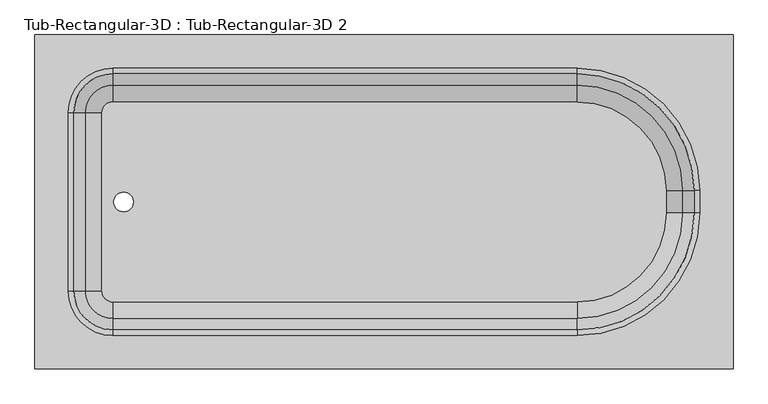
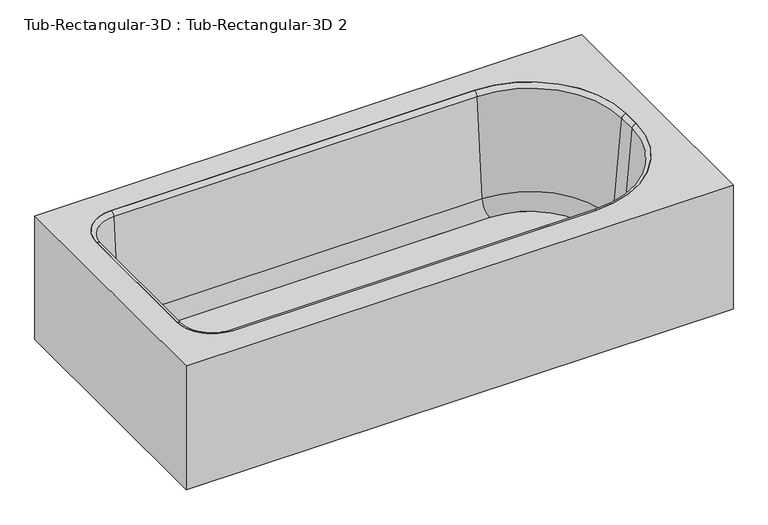
"""IFC4 building model written with IfcOpenShell, lengths in millimetres: flow terminal geometry, Tub-Rectangular-3D : Tub-Rectangular-3D 2."""

from ifc_helpers import new_model, si_unit, point, frame, frame_2d, origin, place, context, project, spatial, polyline, circle_curve, ellipse_curve, trimmed, segment, composite_curve, outline, extrude, source, transform, mapped, element, save
from ifc_brep_helpers import plane_surface, cylinder_surface, revolved_surface, advanced_brep


def tub_rectangular_3d_tub_rectangular_3d_2_4c7bd2b7(model_context):
    return source(origin(), model_context, "Body", "SolidModel", [
        advanced_brep(
        [(480.0720313, 866.775, 381.0), (-1110.6029687, 866.775, 381.0), (-1110.6029687, 104.775, 381.0), (480.0720313, 104.775, 381.0), (-932.8029687, 790.575, 381.0), (124.4720313, 790.575, 381.0), (403.8720313, 511.175, 381.0), (403.8720313, 460.375, 381.0), (124.4720313, 180.975, 381.0), (-932.8029687, 180.975, 381.0), (-1034.4029687, 282.575, 381.0), (-1034.4029687, 688.975, 381.0), (461.0220313, 847.725, 361.95), (461.0220313, 123.825, 361.95), (-1091.5529687, 123.825, 361.95), (-1091.5529687, 847.725, 361.95), (-932.8029687, 790.575, 361.95), (-1034.4029687, 688.975, 361.95), (-1034.4029687, 282.575, 361.95), (-932.8029687, 180.975, 361.95), (124.4720313, 180.975, 361.95), (403.8720313, 460.375, 361.95), (403.8720313, 511.175, 361.95), (124.4720313, 790.575, 361.95), (480.0720313, 866.775, 0.0), (-1110.6029687, 866.775, 0.0), (-1110.6029687, 104.775, 0.0), (480.0720313, 104.775, 0.0), (461.0220313, 847.725, 0.0), (-1091.5529687, 847.725, 0.0), (-1091.5529687, 123.825, 0.0), (461.0220313, 123.825, 0.0)],
        [
            (0, 1),
            (1, 2),
            (2, 3),
            (3, 0),
            (4, 5),
            (5, 6, circle_curve(frame((124.4720313, 511.175, 381.0), z_axis=(0.0, 0.0, -1.0), x_axis=(0.0, 1.0, 0.0)), 279.4)),
            (6, 7),
            (7, 8, circle_curve(frame((124.4720313, 460.375, 381.0), z_axis=(0.0, 0.0, -1.0), x_axis=(0.0, 1.0, 0.0)), 279.4)),
            (8, 9),
            (9, 10, circle_curve(frame((-932.8029687, 282.575, 381.0), z_axis=(0.0, 0.0, -1.0), x_axis=(0.0, 1.0, 0.0)), 101.6)),
            (10, 11),
            (11, 4, circle_curve(frame((-932.8029687, 688.975, 381.0), z_axis=(0.0, 0.0, -1.0), x_axis=(0.0, 1.0, 0.0)), 101.6)),
            (12, 13),
            (13, 14),
            (14, 15),
            (15, 12),
            (16, 17, circle_curve(frame((-932.8029687, 688.975, 361.95), z_axis=(0.0, 0.0, 1.0), x_axis=(0.0, 1.0, 0.0)), 101.6)),
            (17, 18),
            (18, 19, circle_curve(frame((-932.8029687, 282.575, 361.95), z_axis=(0.0, 0.0, 1.0), x_axis=(0.0, 1.0, 0.0)), 101.6)),
            (19, 20),
            (20, 21, circle_curve(frame((124.4720313, 460.375, 361.95), z_axis=(0.0, 0.0, 1.0), x_axis=(0.0, 1.0, 0.0)), 279.4)),
            (21, 22),
            (22, 23, circle_curve(frame((124.4720313, 511.175, 361.95), z_axis=(0.0, 0.0, 1.0), x_axis=(0.0, 1.0, 0.0)), 279.4)),
            (23, 16),
            (0, 24),
            (24, 25),
            (25, 1),
            (25, 26),
            (26, 2),
            (26, 27),
            (27, 3),
            (27, 24),
            (4, 16),
            (23, 5),
            (22, 6),
            (21, 7),
            (20, 8),
            (19, 9),
            (18, 10),
            (17, 11),
            (28, 29),
            (29, 30),
            (30, 31),
            (31, 28),
            (31, 13),
            (12, 28),
            (30, 14),
            (29, 15),
        ],
        [
            plane_surface(frame((-1110.6029687, 866.775, 381.0), z_axis=(0.0, 0.0, 1.0), x_axis=(-1.0, 0.0, 0.0))),
            plane_surface(frame((-1110.6029687, 866.775, 361.95), z_axis=(0.0, 0.0, -1.0), x_axis=(1.0, 0.0, 0.0))),
            plane_surface(frame((480.0720313, 866.775, 381.0), z_axis=(0.0, 1.0, 0.0), x_axis=(0.0, 0.0, -1.0))),
            plane_surface(frame((-1110.6029687, 866.775, 381.0), z_axis=(-1.0, 0.0, 0.0), x_axis=(0.0, 0.0, -1.0))),
            plane_surface(frame((-1110.6029687, 104.775, 381.0), z_axis=(0.0, -1.0, 0.0), x_axis=(0.0, 0.0, -1.0))),
            plane_surface(frame((480.0720313, 104.775, 381.0), z_axis=(1.0, 0.0, 0.0), x_axis=(0.0, 0.0, -1.0))),
            plane_surface(frame((-932.8029687, 790.575, 381.0), z_axis=(0.0, -1.0, 0.0), x_axis=(0.0, 0.0, -1.0))),
            revolved_surface(polyline([(124.4720313, 790.575, 361.95), (124.4720313, 790.575, 381.0)]), (124.4720313, 511.175, 381.0), (0.0, 0.0, -1.0)),
            plane_surface(frame((403.8720313, 511.175, 381.0), z_axis=(-1.0, 0.0, 0.0), x_axis=(0.0, 0.0, -1.0))),
            revolved_surface(polyline([(124.4720313, 739.775, 361.95), (124.4720313, 739.775, 381.0)]), (124.4720313, 460.375, 381.0), (0.0, 0.0, -1.0)),
            plane_surface(frame((124.4720313, 180.975, 381.0), z_axis=(0.0, 1.0, 0.0), x_axis=(0.0, 0.0, -1.0))),
            revolved_surface(polyline([(-932.8029687, 384.17499999999995, 361.95), (-932.8029687, 384.17499999999995, 381.0)]), (-932.8029687, 282.575, 381.0), (0.0, 0.0, -1.0)),
            plane_surface(frame((-1034.4029687, 282.575, 381.0), z_axis=(1.0, 0.0, 0.0), x_axis=(0.0, 0.0, -1.0))),
            revolved_surface(polyline([(-932.8029687, 790.575, 361.95), (-932.8029687, 790.575, 381.0)]), (-932.8029687, 688.975, 381.0), (0.0, 0.0, -1.0)),
            plane_surface(frame((-1110.6029687, 866.775, 0.0), z_axis=(0.0, 0.0, -1.0), x_axis=(1.0, 0.0, 0.0))),
            plane_surface(frame((461.0220313, 847.725, 361.95), z_axis=(-1.0, 0.0, 0.0), x_axis=(0.0, 0.0, -1.0))),
            plane_surface(frame((461.0220313, 123.825, 361.95), z_axis=(0.0, 1.0, 0.0), x_axis=(0.0, 0.0, -1.0))),
            plane_surface(frame((-1091.5529687, 123.825, 361.95), z_axis=(1.0, 0.0, 0.0), x_axis=(0.0, 0.0, -1.0))),
            plane_surface(frame((-1091.5529687, 847.725, 361.95), z_axis=(0.0, -1.0, 0.0), x_axis=(0.0, 0.0, -1.0))),
        ],
        [
            (0, [[1, 2, 3, 4], [5, 6, 7, 8, 9, 10, 11, 12]]),
            (1, [[13, 14, 15, 16], [17, 18, 19, 20, 21, 22, 23, 24]]),
            (2, [[-1, 25, 26, 27]]),
            (3, [[-2, -27, 28, 29]]),
            (4, [[-3, -29, 30, 31]]),
            (5, [[-25, -4, -31, 32]]),
            (6, [[-5, 33, -24, 34]]),
            (7, [[-6, -34, -23, 35]]),
            (8, [[-7, -35, -22, 36]]),
            (9, [[-8, -36, -21, 37]]),
            (10, [[-9, -37, -20, 38]]),
            (11, [[-10, -38, -19, 39]]),
            (12, [[-11, -39, -18, 40]]),
            (13, [[-12, -40, -17, -33]]),
            (14, [[-32, -30, -28, -26], [41, 42, 43, 44]]),
            (15, [[-44, 45, -13, 46]]),
            (16, [[-43, 47, -14, -45]]),
            (17, [[-42, 48, -15, -47]]),
            (18, [[-41, -46, -16, -48]]),
        ],
    ),
        extrude(outline(composite_curve([segment(trimmed(circle_curve(frame_2d((124.4720313, 511.175)), 202.7964741), [point((124.4720313, 713.9714741))], [point((327.2685054, 511.175))], False, "CARTESIAN"), True, "CONTINUOUS"), segment(polyline([(327.2685054, 511.175), (327.2685054, 460.375)]), True, "CONTINUOUS"), segment(trimmed(circle_curve(frame_2d((124.4720313, 460.375)), 202.7964741), [point((327.2685054, 460.375))], [point((124.4720313, 257.5785259))], False, "CARTESIAN"), True, "CONTINUOUS"), segment(polyline([(124.4720313, 257.5785259), (-932.8029687, 257.5785259)]), True, "CONTINUOUS"), segment(trimmed(circle_curve(frame_2d((-932.8029687, 282.575)), 24.9964741), [point((-932.8029687, 257.5785259))], [point((-957.7994428, 282.575))], False, "CARTESIAN"), True, "CONTINUOUS"), segment(polyline([(-957.7994428, 282.575), (-957.7994428, 688.975)]), True, "CONTINUOUS"), segment(trimmed(circle_curve(frame_2d((-932.8029687, 688.975)), 24.9964741), [point((-957.7994428, 688.975))], [point((-932.8029687, 713.9714741))], False, "CARTESIAN"), True, "CONTINUOUS"), segment(polyline([(-932.8029687, 713.9714741), (124.4720313, 713.9714741)]), True, "CONTINUOUS")], self_intersect=False), holes=[composite_curve([segment(trimmed(circle_curve(frame_2d((-908.510206, 485.775)), 22.225), [point((-908.510206, 508.0))], [point((-908.510206, 463.55))], True, "CARTESIAN"), True, "CONTINUOUS"), segment(trimmed(circle_curve(frame_2d((-908.510206, 485.775)), 22.225), [point((-908.510206, 463.55))], [point((-908.510206, 508.0))], True, "CARTESIAN"), True, "CONTINUOUS")], self_intersect=False)]), frame((0.0, 0.0, 16.863573), z_axis=(0.0, 0.0, 1.0), x_axis=(1.0, 0.0, 0.0)), (0.0, 0.0, 1.0), 19.05),
        advanced_brep(
        [(-995.7544608, 688.975, 70.6929392), (-932.8029687, 751.9264921, 70.6929392), (-932.8029687, 778.0970035, 369.8232535), (-1021.9249722, 688.975, 369.8232535), (-957.7994428, 688.975, 35.913573), (-932.8029687, 713.9714741, 35.913573), (-957.7994428, 688.975, 16.863573), (-932.8029687, 713.9714741, 16.863573), (-1034.4029687, 688.975, 16.863573), (-932.8029687, 790.575, 16.863573), (-1034.4029687, 688.975, 381.0), (-932.8029687, 790.575, 381.0), (-1021.9249722, 282.575, 369.8232535), (-995.7544608, 282.575, 70.6929392), (-957.7994428, 282.575, 35.913573), (-957.7994428, 282.575, 16.863573), (-1034.4029687, 282.575, 16.863573), (-1034.4029687, 282.575, 381.0), (-932.8029687, 219.6235079, 70.6929392), (-932.8029687, 193.4529965, 369.8232535), (-932.8029687, 257.5785259, 35.913573), (-932.8029687, 257.5785259, 16.863573), (-932.8029687, 180.975, 16.863573), (-932.8029687, 180.975, 381.0), (124.4720313, 193.4529965, 369.8232535), (124.4720313, 219.6235079, 70.6929392), (124.4720313, 257.5785259, 35.913573), (124.4720313, 257.5785259, 16.863573), (124.4720313, 180.975, 16.863573), (124.4720313, 180.975, 381.0), (365.2235234, 460.375, 70.6929392), (391.3940348, 460.375, 369.8232535), (327.2685054, 460.375, 35.913573), (327.2685054, 460.375, 16.863573), (403.8720313, 460.375, 16.863573), (403.8720313, 460.375, 381.0), (391.3940348, 511.175, 369.8232535), (365.2235234, 511.175, 70.6929392), (327.2685054, 511.175, 35.913573), (327.2685054, 511.175, 16.863573), (403.8720313, 511.175, 16.863573), (403.8720313, 511.175, 381.0), (124.4720313, 751.9264921, 70.6929392), (124.4720313, 778.0970035, 369.8232535), (124.4720313, 713.9714741, 35.913573), (124.4720313, 713.9714741, 16.863573), (124.4720313, 790.575, 16.863573), (124.4720313, 790.575, 381.0)],
        [
            (0, 1, circle_curve(frame((-932.8029687, 688.975, 70.6929392), z_axis=(0.0, 0.0, -1.0), x_axis=(0.0, 1.0, 0.0)), 62.9514921)),
            (1, 2),
            (2, 3, circle_curve(frame((-932.8029687, 688.975, 369.8232535), z_axis=(0.0, 0.0, 1.0), x_axis=(0.0, 1.0, 0.0)), 89.1220035)),
            (3, 0),
            (4, 5, circle_curve(frame((-932.8029687, 688.975, 35.913573), z_axis=(0.0, 0.0, -1.0), x_axis=(0.0, 1.0, 0.0)), 24.9964741)),
            (5, 1, circle_curve(frame((-932.8029687, 713.9714741, 74.013573), z_axis=(1.0, 0.0, 0.0), x_axis=(0.0, -1.0, 0.0)), 38.1)),
            (0, 4, circle_curve(frame((-957.7994428, 688.975, 74.013573), z_axis=(0.0, -1.0, 0.0), x_axis=(1.0, 0.0, 0.0)), 38.1)),
            (6, 7, circle_curve(frame((-932.8029687, 688.975, 16.863573), z_axis=(0.0, 0.0, -1.0), x_axis=(0.0, 1.0, 0.0)), 24.9964741)),
            (7, 5),
            (4, 6),
            (8, 9, circle_curve(frame((-932.8029687, 688.975, 16.863573), z_axis=(0.0, 0.0, -1.0), x_axis=(0.0, 1.0, 0.0)), 101.6)),
            (9, 7),
            (6, 8),
            (10, 11, circle_curve(frame((-932.8029687, 688.975, 381.0), z_axis=(0.0, 0.0, -1.0), x_axis=(0.0, 1.0, 0.0)), 101.6)),
            (11, 9),
            (8, 10),
            (2, 11, circle_curve(frame((-932.8029687, 790.575, 368.4462547), z_axis=(-1.0, 0.0, 0.0), x_axis=(0.0, -1.0, 0.0)), 12.5537453)),
            (10, 3, circle_curve(frame((-1034.4029687, 688.975, 368.4462547), z_axis=(0.0, 1.0, 0.0), x_axis=(1.0, 0.0, 0.0)), 12.5537453)),
            (3, 12),
            (12, 13),
            (13, 0),
            (13, 14, circle_curve(frame((-957.7994428, 282.575, 74.013573), z_axis=(0.0, -1.0, 0.0), x_axis=(1.0, 0.0, 0.0)), 38.1)),
            (14, 4),
            (14, 15),
            (15, 6),
            (15, 16),
            (16, 8),
            (16, 17),
            (17, 10),
            (17, 12, circle_curve(frame((-1034.4029687, 282.575, 368.4462547), z_axis=(0.0, 1.0, 0.0), x_axis=(1.0, 0.0, 0.0)), 12.5537453)),
            (18, 13, circle_curve(frame((-932.8029687, 282.575, 70.6929392), z_axis=(0.0, 0.0, -1.0), x_axis=(-1.0, 0.0, 0.0)), 62.9514921)),
            (12, 19, circle_curve(frame((-932.8029687, 282.575, 369.8232535), z_axis=(0.0, 0.0, 1.0), x_axis=(-1.0, 0.0, 0.0)), 89.1220035)),
            (19, 18),
            (20, 14, circle_curve(frame((-932.8029687, 282.575, 35.913573), z_axis=(0.0, 0.0, -1.0), x_axis=(-1.0, 0.0, 0.0)), 24.9964741)),
            (18, 20, circle_curve(frame((-932.8029687, 257.5785259, 74.013573), z_axis=(1.0, 0.0, 0.0), x_axis=(0.0, 1.0, 0.0)), 38.1)),
            (21, 15, circle_curve(frame((-932.8029687, 282.575, 16.863573), z_axis=(0.0, 0.0, -1.0), x_axis=(-1.0, 0.0, 0.0)), 24.9964741)),
            (20, 21),
            (22, 16, circle_curve(frame((-932.8029687, 282.575, 16.863573), z_axis=(0.0, 0.0, -1.0), x_axis=(-1.0, 0.0, 0.0)), 101.6)),
            (21, 22),
            (23, 17, circle_curve(frame((-932.8029687, 282.575, 381.0), z_axis=(0.0, 0.0, -1.0), x_axis=(-1.0, 0.0, 0.0)), 101.6)),
            (22, 23),
            (23, 19, circle_curve(frame((-932.8029687, 180.975, 368.4462547), z_axis=(-1.0, 0.0, 0.0), x_axis=(0.0, 1.0, 0.0)), 12.5537453)),
            (19, 24),
            (24, 25),
            (25, 18),
            (25, 26, circle_curve(frame((124.4720313, 257.5785259, 74.013573), z_axis=(1.0, 0.0, 0.0), x_axis=(0.0, 1.0, 0.0)), 38.1)),
            (26, 20),
            (26, 27),
            (27, 21),
            (27, 28),
            (28, 22),
            (28, 29),
            (29, 23),
            (29, 24, circle_curve(frame((124.4720313, 180.975, 368.4462547), z_axis=(-1.0, 0.0, 0.0), x_axis=(0.0, 1.0, 0.0)), 12.5537453)),
            (30, 25, circle_curve(frame((124.4720313, 460.375, 70.6929392), z_axis=(0.0, 0.0, -1.0), x_axis=(0.0, -1.0, 0.0)), 240.7514921)),
            (24, 31, circle_curve(frame((124.4720313, 460.375, 369.8232535), z_axis=(0.0, 0.0, 1.0), x_axis=(0.0, -1.0, 0.0)), 266.9220035)),
            (31, 30),
            (32, 26, circle_curve(frame((124.4720313, 460.375, 35.913573), z_axis=(0.0, 0.0, -1.0), x_axis=(0.0, -1.0, 0.0)), 202.7964741)),
            (30, 32, circle_curve(frame((327.2685054, 460.375, 74.013573), z_axis=(0.0, 1.0, 0.0), x_axis=(-1.0, 0.0, 0.0)), 38.1)),
            (33, 27, circle_curve(frame((124.4720313, 460.375, 16.863573), z_axis=(0.0, 0.0, -1.0), x_axis=(0.0, -1.0, 0.0)), 202.7964741)),
            (32, 33),
            (34, 28, circle_curve(frame((124.4720313, 460.375, 16.863573), z_axis=(0.0, 0.0, -1.0), x_axis=(0.0, -1.0, 0.0)), 279.4)),
            (33, 34),
            (35, 29, circle_curve(frame((124.4720313, 460.375, 381.0), z_axis=(0.0, 0.0, -1.0), x_axis=(0.0, -1.0, 0.0)), 279.4)),
            (34, 35),
            (35, 31, circle_curve(frame((403.8720313, 460.375, 368.4462547), z_axis=(0.0, -1.0, 0.0), x_axis=(-1.0, 0.0, 0.0)), 12.5537453)),
            (31, 36),
            (36, 37),
            (37, 30),
            (37, 38, circle_curve(frame((327.2685054, 511.175, 74.013573), z_axis=(0.0, 1.0, 0.0), x_axis=(-1.0, 0.0, 0.0)), 38.1)),
            (38, 32),
            (38, 39),
            (39, 33),
            (39, 40),
            (40, 34),
            (40, 41),
            (41, 35),
            (41, 36, circle_curve(frame((403.8720313, 511.175, 368.4462547), z_axis=(0.0, -1.0, 0.0), x_axis=(-1.0, 0.0, 0.0)), 12.5537453)),
            (42, 37, circle_curve(frame((124.4720313, 511.175, 70.6929392), z_axis=(0.0, 0.0, -1.0), x_axis=(1.0, 0.0, 0.0)), 240.7514921)),
            (36, 43, circle_curve(frame((124.4720313, 511.175, 369.8232535), z_axis=(0.0, 0.0, 1.0), x_axis=(1.0, 0.0, 0.0)), 266.9220035)),
            (43, 42),
            (44, 38, circle_curve(frame((124.4720313, 511.175, 35.913573), z_axis=(0.0, 0.0, -1.0), x_axis=(1.0, 0.0, 0.0)), 202.7964741)),
            (42, 44, circle_curve(frame((124.4720313, 713.9714741, 74.013573), z_axis=(-1.0, 0.0, 0.0), x_axis=(0.0, -1.0, 0.0)), 38.1)),
            (45, 39, circle_curve(frame((124.4720313, 511.175, 16.863573), z_axis=(0.0, 0.0, -1.0), x_axis=(1.0, 0.0, 0.0)), 202.7964741)),
            (44, 45),
            (46, 40, circle_curve(frame((124.4720313, 511.175, 16.863573), z_axis=(0.0, 0.0, -1.0), x_axis=(1.0, 0.0, 0.0)), 279.4)),
            (45, 46),
            (47, 41, circle_curve(frame((124.4720313, 511.175, 381.0), z_axis=(0.0, 0.0, -1.0), x_axis=(1.0, 0.0, 0.0)), 279.4)),
            (46, 47),
            (47, 43, circle_curve(frame((124.4720313, 790.575, 368.4462547), z_axis=(1.0, 0.0, 0.0), x_axis=(0.0, -1.0, 0.0)), 12.5537453)),
            (43, 2),
            (1, 42),
            (5, 44),
            (7, 45),
            (9, 46),
            (11, 47),
        ],
        [
            revolved_surface(polyline([(-932.8029687, 778.0970035, 369.8232535), (-932.8029687, 751.9264921, 70.6929392)]), (-932.8029687, 688.975, 381.0), (0.0, 0.0, 1.0)),
            revolved_surface(trimmed(ellipse_curve(frame((-932.8029687, 713.9714741, 74.013573), z_axis=(-1.0, 0.0, 0.0), x_axis=(0.0, -1.0, 0.0)), 38.1, 38.1), [point((-932.8029687, 751.9264921, 70.6929392))], [point((-932.8029687, 713.9714741, 35.913573))], True, "CARTESIAN"), (-932.8029687, 688.975, 381.0), (0.0, 0.0, 1.0)),
            revolved_surface(polyline([(-932.8029687, 713.9714741, 35.913572999999985), (-932.8029687, 713.9714741, 16.863572999999974)]), (-932.8029687, 688.975, 381.0), (0.0, 0.0, 1.0)),
            plane_surface(frame((-932.8029687, 688.975, 16.863573), z_axis=(0.0, 0.0, -1.0), x_axis=(0.0, 1.0, 0.0))),
            cylinder_surface(frame((-932.8029687, 688.975, 381.0), z_axis=(0.0, 0.0, 1.0), x_axis=(0.0, 1.0, 0.0)), 101.6),
            revolved_surface(trimmed(ellipse_curve(frame((-932.8029687, 790.575, 368.4462547), z_axis=(1.0, 0.0, 0.0), x_axis=(0.0, -1.0, 0.0)), 12.5537453, 12.5537453), [point((-932.8029687, 790.575, 381.0))], [point((-932.8029687, 778.0970035, 369.8232535))], True, "CARTESIAN"), (-932.8029687, 688.975, 381.0), (0.0, 0.0, 1.0)),
            plane_surface(frame((-1021.9249722, 688.975, 369.8232535), z_axis=(0.9961946980917458, 0.0, 0.08715574274765597), x_axis=(0.0, -1.0, 0.0))),
            revolved_surface(polyline([(-919.6994427999999, 282.575, 74.013573), (-919.6994427999999, 688.975, 74.013573)]), (-957.7994428, 688.975, 74.013573), (0.0, -1.0, 0.0)),
            plane_surface(frame((-957.7994428, 688.975, 35.913573), z_axis=(1.0, 0.0, 0.0), x_axis=(0.0, -1.0, 0.0))),
            plane_surface(frame((-957.7994428, 688.975, 16.863573), z_axis=(0.0, 0.0, -1.0), x_axis=(0.0, -1.0, 0.0))),
            plane_surface(frame((-1034.4029687, 688.975, 16.863573), z_axis=(-1.0, 0.0, 0.0), x_axis=(0.0, -1.0, 0.0))),
            cylinder_surface(frame((-1034.4029687, 688.975, 368.4462547), z_axis=(0.0, 1.0, 0.0), x_axis=(1.0, 0.0, 0.0)), 12.5537453),
            revolved_surface(polyline([(-1021.9249722, 282.575, 369.8232535), (-995.7544608, 282.575, 70.6929392)]), (-932.8029687, 282.575, 381.0), (0.0, 0.0, 1.0)),
            revolved_surface(trimmed(ellipse_curve(frame((-957.7994428, 282.575, 74.013573), z_axis=(0.0, -1.0, 0.0), x_axis=(1.0, 0.0, 0.0)), 38.1, 38.1), [point((-995.7544608, 282.575, 70.6929392))], [point((-957.7994428, 282.575, 35.913573))], True, "CARTESIAN"), (-932.8029687, 282.575, 381.0), (0.0, 0.0, 1.0)),
            revolved_surface(polyline([(-957.7994428, 282.575, 35.913572999999985), (-957.7994428, 282.575, 16.863572999999974)]), (-932.8029687, 282.575, 381.0), (0.0, 0.0, 1.0)),
            plane_surface(frame((-932.8029687, 282.575, 16.863573), z_axis=(0.0, 0.0, -1.0), x_axis=(-1.0, 0.0, 0.0))),
            cylinder_surface(frame((-932.8029687, 282.575, 381.0), z_axis=(0.0, 0.0, 1.0), x_axis=(-1.0, 0.0, 0.0)), 101.6),
            revolved_surface(trimmed(ellipse_curve(frame((-1034.4029687, 282.575, 368.4462547), z_axis=(0.0, 1.0, 0.0), x_axis=(1.0, 0.0, 0.0)), 12.5537453, 12.5537453), [point((-1034.4029687, 282.575, 381.0))], [point((-1021.9249722, 282.575, 369.8232535))], True, "CARTESIAN"), (-932.8029687, 282.575, 381.0), (0.0, 0.0, 1.0)),
            plane_surface(frame((-932.8029687, 193.4529965, 369.8232535), z_axis=(0.0, 0.9961946980917461, 0.08715574274765274), x_axis=(1.0, 0.0, 0.0))),
            revolved_surface(polyline([(124.47203129999991, 295.6785259, 74.013573), (-932.8029687, 295.6785259, 74.013573)]), (-932.8029687, 257.5785259, 74.013573), (1.0, 0.0, 0.0)),
            plane_surface(frame((-932.8029687, 257.5785259, 35.913573), z_axis=(0.0, 1.0, 0.0), x_axis=(1.0, 0.0, 0.0))),
            plane_surface(frame((-932.8029687, 257.5785259, 16.863573), z_axis=(0.0, 0.0, -1.0), x_axis=(1.0, 0.0, 0.0))),
            plane_surface(frame((-932.8029687, 180.975, 16.863573), z_axis=(0.0, -1.0, 0.0), x_axis=(1.0, 0.0, 0.0))),
            cylinder_surface(frame((-932.8029687, 180.975, 368.4462547), z_axis=(-1.0, 0.0, 0.0), x_axis=(0.0, 1.0, 0.0)), 12.5537453),
            revolved_surface(polyline([(124.4720313, 193.4529965, 369.8232535), (124.4720313, 219.6235079, 70.6929392)]), (124.4720313, 460.375, 381.0), (0.0, 0.0, 1.0)),
            revolved_surface(trimmed(ellipse_curve(frame((124.4720313, 257.5785259, 74.013573), z_axis=(1.0, 0.0, 0.0), x_axis=(0.0, 1.0, 0.0)), 38.1, 38.1), [point((124.4720313, 219.6235079, 70.6929392))], [point((124.4720313, 257.5785259, 35.913573))], True, "CARTESIAN"), (124.4720313, 460.375, 381.0), (0.0, 0.0, 1.0)),
            revolved_surface(polyline([(124.4720313, 257.5785259, 35.913572999999985), (124.4720313, 257.5785259, 16.863572999999974)]), (124.4720313, 460.375, 381.0), (0.0, 0.0, 1.0)),
            plane_surface(frame((124.4720313, 460.375, 16.863573), z_axis=(0.0, 0.0, -1.0), x_axis=(0.0, -1.0, 0.0))),
            cylinder_surface(frame((124.4720313, 460.375, 381.0), z_axis=(0.0, 0.0, 1.0), x_axis=(0.0, -1.0, 0.0)), 279.4),
            revolved_surface(trimmed(ellipse_curve(frame((124.4720313, 180.975, 368.4462547), z_axis=(-1.0, 0.0, 0.0), x_axis=(0.0, 1.0, 0.0)), 12.5537453, 12.5537453), [point((124.4720313, 180.975, 381.0))], [point((124.4720313, 193.4529965, 369.8232535))], True, "CARTESIAN"), (124.4720313, 460.375, 381.0), (0.0, 0.0, 1.0)),
            plane_surface(frame((391.3940348, 460.375, 369.8232535), z_axis=(-0.9961946980917464, 0.0, 0.0871557427476495), x_axis=(0.0, 1.0, 0.0))),
            revolved_surface(polyline([(289.16850539999996, 511.175, 74.013573), (289.16850539999996, 460.375, 74.013573)]), (327.2685054, 460.375, 74.013573), (0.0, 1.0, 0.0)),
            plane_surface(frame((327.2685054, 460.375, 35.913573), z_axis=(-1.0, 0.0, 0.0), x_axis=(0.0, 1.0, 0.0))),
            plane_surface(frame((327.2685054, 460.375, 16.863573), z_axis=(0.0, 0.0, -1.0), x_axis=(0.0, 1.0, 0.0))),
            plane_surface(frame((403.8720313, 460.375, 16.863573), z_axis=(1.0, 0.0, 0.0), x_axis=(0.0, 1.0, 0.0))),
            cylinder_surface(frame((403.8720313, 460.375, 368.4462547), z_axis=(0.0, -1.0, 0.0), x_axis=(-1.0, 0.0, 0.0)), 12.5537453),
            revolved_surface(polyline([(391.3940348, 511.175, 369.8232535), (365.2235234, 511.175, 70.6929392)]), (124.4720313, 511.175, 381.0), (0.0, 0.0, 1.0)),
            revolved_surface(trimmed(ellipse_curve(frame((327.2685054, 511.175, 74.013573), z_axis=(0.0, 1.0, 0.0), x_axis=(-1.0, 0.0, 0.0)), 38.1, 38.1), [point((365.2235234, 511.175, 70.6929392))], [point((327.2685054, 511.175, 35.913573))], True, "CARTESIAN"), (124.4720313, 511.175, 381.0), (0.0, 0.0, 1.0)),
            revolved_surface(polyline([(327.2685054, 511.175, 35.913572999999985), (327.2685054, 511.175, 16.863572999999974)]), (124.4720313, 511.175, 381.0), (0.0, 0.0, 1.0)),
            plane_surface(frame((124.4720313, 511.175, 16.863573), z_axis=(0.0, 0.0, -1.0), x_axis=(1.0, 0.0, 0.0))),
            cylinder_surface(frame((124.4720313, 511.175, 381.0), z_axis=(0.0, 0.0, 1.0), x_axis=(1.0, 0.0, 0.0)), 279.4),
            revolved_surface(trimmed(ellipse_curve(frame((403.8720313, 511.175, 368.4462547), z_axis=(0.0, -1.0, 0.0), x_axis=(-1.0, 0.0, 0.0)), 12.5537453, 12.5537453), [point((403.8720313, 511.175, 381.0))], [point((391.3940348, 511.175, 369.8232535))], True, "CARTESIAN"), (124.4720313, 511.175, 381.0), (0.0, 0.0, 1.0)),
            plane_surface(frame((124.4720313, 778.0970035, 369.8232535), z_axis=(0.0, -0.9961946980917461, 0.08715574274765274), x_axis=(-1.0, 0.0, 0.0))),
            revolved_surface(polyline([(-932.8029686999998, 675.8714741, 74.013573), (124.4720313, 675.8714741, 74.013573)]), (124.4720313, 713.9714741, 74.013573), (-1.0, 0.0, 0.0)),
            plane_surface(frame((124.4720313, 713.9714741, 35.913573), z_axis=(0.0, -1.0, 0.0), x_axis=(-1.0, 0.0, 0.0))),
            plane_surface(frame((124.4720313, 713.9714741, 16.863573), z_axis=(0.0, 0.0, -1.0), x_axis=(-1.0, 0.0, 0.0))),
            plane_surface(frame((124.4720313, 790.575, 16.863573), z_axis=(0.0, 1.0, 0.0), x_axis=(-1.0, 0.0, 0.0))),
            cylinder_surface(frame((124.4720313, 790.575, 368.4462547), z_axis=(1.0, 0.0, 0.0), x_axis=(0.0, -1.0, 0.0)), 12.5537453),
        ],
        [
            (0, [[1, 2, 3, 4]]),
            (1, [[5, 6, -1, 7]]),
            (2, [[8, 9, -5, 10]]),
            (3, [[11, 12, -8, 13]]),
            (4, [[14, 15, -11, 16]]),
            (5, [[-3, 17, -14, 18]]),
            (6, [[-4, 19, 20, 21]]),
            (7, [[-7, -21, 22, 23]]),
            (8, [[-10, -23, 24, 25]]),
            (9, [[-13, -25, 26, 27]]),
            (10, [[-16, -27, 28, 29]]),
            (11, [[-18, -29, 30, -19]]),
            (12, [[31, -20, 32, 33]]),
            (13, [[34, -22, -31, 35]]),
            (14, [[36, -24, -34, 37]]),
            (15, [[38, -26, -36, 39]]),
            (16, [[40, -28, -38, 41]]),
            (17, [[-32, -30, -40, 42]]),
            (18, [[-33, 43, 44, 45]]),
            (19, [[-35, -45, 46, 47]]),
            (20, [[-37, -47, 48, 49]]),
            (21, [[-39, -49, 50, 51]]),
            (22, [[-41, -51, 52, 53]]),
            (23, [[-42, -53, 54, -43]]),
            (24, [[55, -44, 56, 57]]),
            (25, [[58, -46, -55, 59]]),
            (26, [[60, -48, -58, 61]]),
            (27, [[62, -50, -60, 63]]),
            (28, [[64, -52, -62, 65]]),
            (29, [[-56, -54, -64, 66]]),
            (30, [[-57, 67, 68, 69]]),
            (31, [[-59, -69, 70, 71]]),
            (32, [[-61, -71, 72, 73]]),
            (33, [[-63, -73, 74, 75]]),
            (34, [[-65, -75, 76, 77]]),
            (35, [[-66, -77, 78, -67]]),
            (36, [[79, -68, 80, 81]]),
            (37, [[82, -70, -79, 83]]),
            (38, [[84, -72, -82, 85]]),
            (39, [[86, -74, -84, 87]]),
            (40, [[88, -76, -86, 89]]),
            (41, [[-80, -78, -88, 90]]),
            (42, [[-81, 91, -2, 92]]),
            (43, [[-83, -92, -6, 93]]),
            (44, [[-85, -93, -9, 94]]),
            (45, [[-87, -94, -12, 95]]),
            (46, [[-89, -95, -15, 96]]),
            (47, [[-90, -96, -17, -91]]),
        ],
    ),
    ])


if __name__ == "__main__":
    model = new_model("IFC4")
    model_context = context("Model", 3, world=origin())
    ifc_project = project(units=[si_unit("LENGTHUNIT", "METRE", prefix="MILLI")], contexts=[model_context])
    site = spatial("IfcSite", under=ifc_project)
    building = spatial("IfcBuilding", under=site)
    placement = place(None, origin())
    tub_rectangular_3d_tub_rectangular_3d_2_shape = tub_rectangular_3d_tub_rectangular_3d_2_4c7bd2b7(model_context)
    element("IfcFlowTerminal", 1, ObjectType="Tub-Rectangular-3D : Tub-Rectangular-3D 2", at=placement, inside=building, context=model_context, shape_type="MappedRepresentation", body=[
        mapped(tub_rectangular_3d_tub_rectangular_3d_2_shape, transform((0.0, 0.0, 0.0), x_axis=(1.0, 0.0, 0.0), y_axis=(0.0, 1.0, 0.0), z_axis=(0.0, 0.0, 1.0))),
    ])
    save(model, "model.ifc")

# Revit data of these elements
# Type "Tub-Rectangular-3D : Tub-Rectangular-3D 2"
#   Assembly Code = "D2010500"
#   Depth = 2' - 6"
#   Height = 1' - 3"
#   Width = 5' - 2 5/8"
#   Tub Material = Porcelain, Ivory
# Element 1 (IfcFlowTerminal, "Tub-Rectangular-3D : Tub-Rectangular-3D 2")
#   Materials on its faces: "Porcelain, Ivory"
# Materials
#   "Porcelain, Ivory": class "Ceramic", colour RGB 247 247 239, transparency 0, Description = "Porcelain, ivory", Cost = 0
